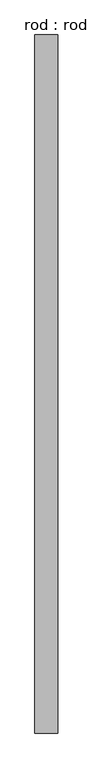
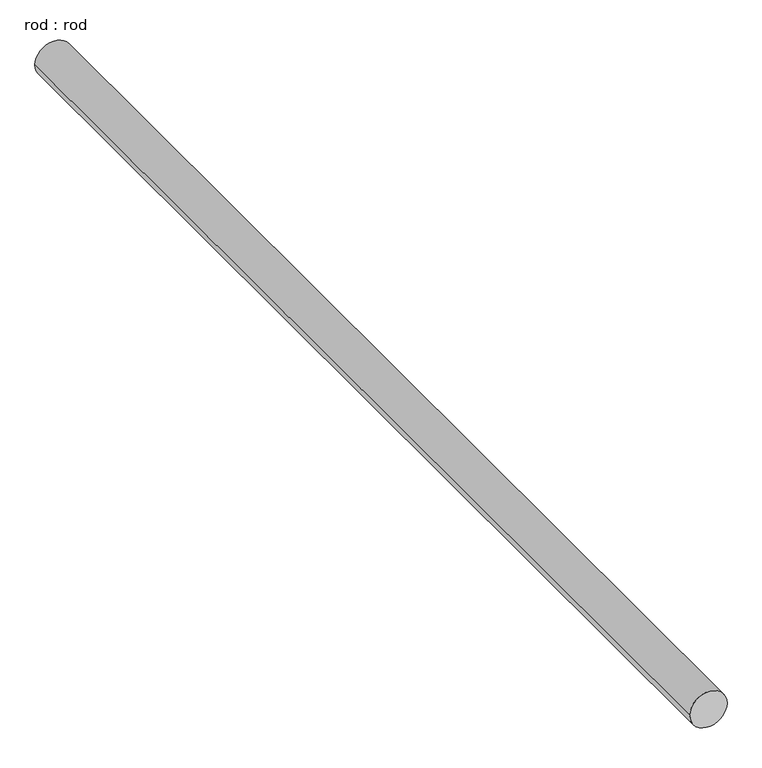
"""IFC4 building model written with IfcOpenShell, lengths in millimetres: proxy geometry, rod : rod."""

from ifc_helpers import new_model, si_unit, point, frame, frame_2d, origin, place, context, project, spatial, circle_curve, trimmed, segment, composite_curve, outline, extrude, source, transform, mapped, element, save


def rod_rod_ead03a13(model_context):
    return source(origin(), model_context, "Body", "SweptSolid", [
        extrude(outline(composite_curve([segment(trimmed(circle_curve(frame_2d((0.0108462, 0.0)), 200.0), [point((0.0108462, 200.0))], [point((0.0108462, -200.0))], False, "CARTESIAN"), True, "CONTINUOUS"), segment(trimmed(circle_curve(frame_2d((0.0108462, 0.0)), 200.0), [point((0.0108462, -200.0))], [point((0.0108462, 200.0))], False, "CARTESIAN"), True, "CONTINUOUS")], self_intersect=False)), frame((0.0, -1979.1799667, 0.0), z_axis=(0.0, 1.0, 0.0), x_axis=(0.0, 0.0, 1.0)), (0.0, 0.0, 1.0), 12143.817164),
    ])


if __name__ == "__main__":
    model = new_model("IFC4")
    model_context = context("Model", 3, world=origin())
    ifc_project = project(units=[si_unit("LENGTHUNIT", "METRE", prefix="MILLI")], contexts=[model_context])
    site = spatial("IfcSite", under=ifc_project)
    building = spatial("IfcBuilding", under=site)
    placement = place(None, origin())
    rod_rod_shape = rod_rod_ead03a13(model_context)
    element("IfcBuildingElementProxy", 1, Name="rod : rod", ObjectType="rod : rod", at=placement, inside=building, context=model_context, shape_type="MappedRepresentation", body=[
        mapped(rod_rod_shape, transform((0.0, 0.0, 0.0), x_axis=(1.0, 0.0, 0.0), y_axis=(0.0, 1.0, 0.0), z_axis=(0.0, 0.0, 1.0))),
    ])
    save(model, "model.ifc")

# Revit data of these elements
# Type "rod : rod"
#   Default Elevation = 0
